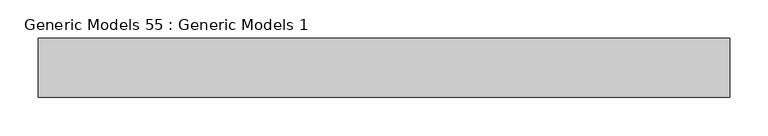
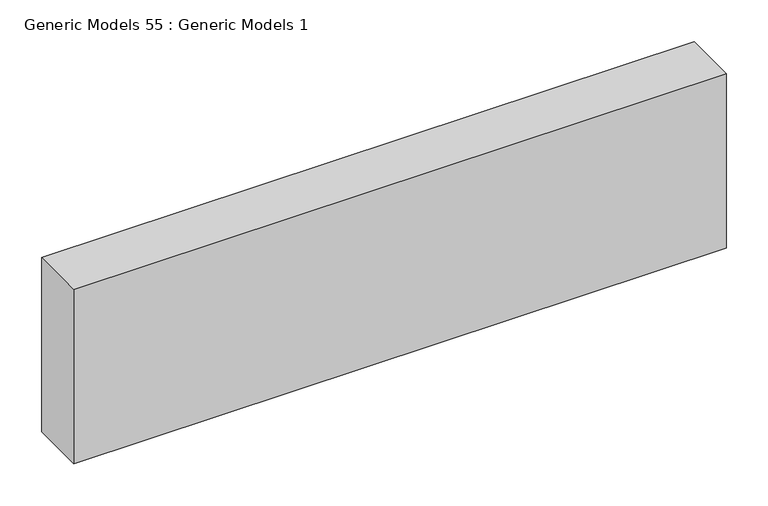
"""IFC4 building model written with IfcOpenShell, lengths in millimetres: proxy geometry, Generic Models 55 : Generic Models 1."""

from ifc_helpers import new_model, si_unit, frame, origin, place, context, project, spatial, polyline, outline, extrude, source, transform, mapped, element, save


def generic_models_55_generic_models_1_d46c6d23(model_context):
    return source(origin(), model_context, "Body", "SweptSolid", [
        extrude(outline(polyline([(-9249.7423796, 482.0227803), (-9249.7423796, 558.2227803), (-8351.6936296, 558.2227803), (-8351.6936296, 482.0227803), (-9249.7423796, 482.0227803)])), frame((0.0, 0.0, 126415.546), z_axis=(0.0, 0.0, 1.0), x_axis=(1.0, 0.0, 0.0)), (0.0, 0.0, 1.0), 254.0),
    ])


if __name__ == "__main__":
    model = new_model("IFC4")
    model_context = context("Model", 3, world=origin())
    ifc_project = project(units=[si_unit("LENGTHUNIT", "METRE", prefix="MILLI")], contexts=[model_context])
    site = spatial("IfcSite", under=ifc_project)
    building = spatial("IfcBuilding", under=site)
    placement = place(None, origin())
    generic_models_55_generic_models_1_shape = generic_models_55_generic_models_1_d46c6d23(model_context)
    element("IfcBuildingElementProxy", 1, Name="Generic Models 55 : Generic Models 1", ObjectType="Generic Models 55 : Generic Models 1", at=placement, inside=building, context=model_context, shape_type="MappedRepresentation", body=[
        mapped(generic_models_55_generic_models_1_shape, transform((0.0, 0.0, 0.0), x_axis=(1.0, 0.0, 0.0), y_axis=(0.0, 1.0, 0.0), z_axis=(0.0, 0.0, 1.0))),
    ])
    save(model, "model.ifc")

# Revit data of these elements
# Element 1 (IfcBuildingElementProxy, "Generic Models 55 : Generic Models 1")
#   Materials on its faces: "_STRUCTURAL MEMBER (SEE STRUCT. DWGS)"
# Materials
#   "_STRUCTURAL MEMBER (SEE STRUCT. DWGS)": class "Generic", colour RGB 209 182 141, transparency 0, Cost = 0
